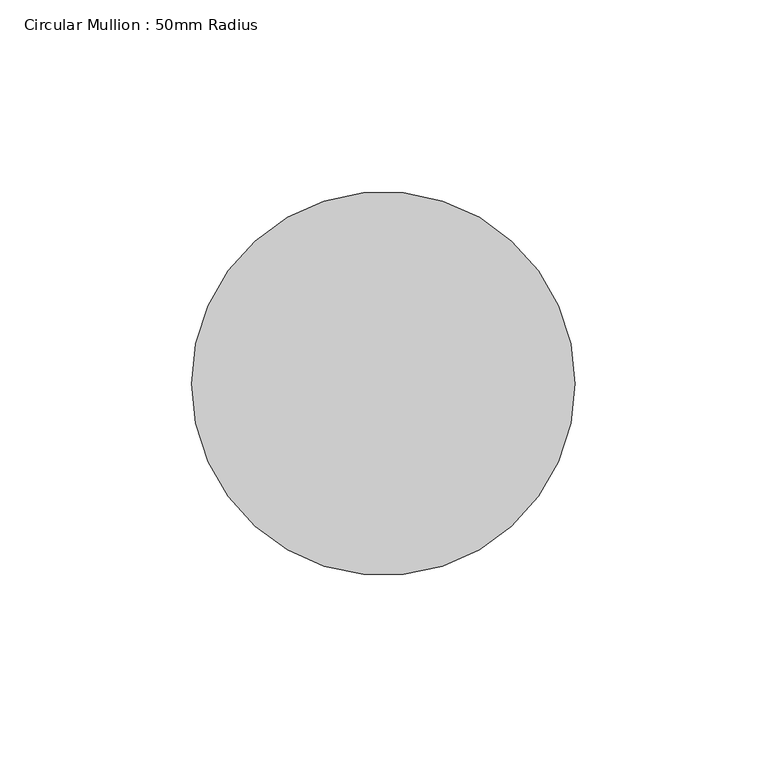
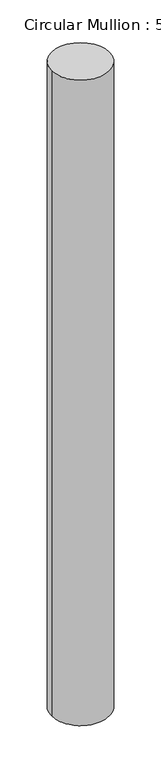
"""IFC4 building model written with IfcOpenShell, lengths in millimetres: member geometry, Circular Mullion : 50mm Radius."""

from ifc_helpers import new_model, si_unit, frame, origin, place, context, project, spatial, ellipse_curve, source, transform, mapped, element, save
from ifc_brep_helpers import plane_surface, cylinder_surface, advanced_brep


def circular_mullion_50mm_radius_35edecd0(model_context):
    return source(origin(), model_context, "Body", "AdvancedBrep", [
        advanced_brep(
        [(-100.0, 0.0, 0.7649818), (0.0, 0.0, 0.0), (0.0, 0.0, -1179.5961113), (-100.0, 0.0, -1180.3293723)],
        [
            (0, 1, ellipse_curve(frame((-50.0, 0.0, 0.3824909), z_axis=(-0.007648899186125256, -0.013483113711122539, -0.9998798427740673), x_axis=(-0.49336672127457615, -0.8696832632198164, 0.015501613274313146)), 50.0060086, 50.0)),
            (1, 2),
            (2, 3, ellipse_curve(frame((-50.0, 0.0, -1179.9627418), z_axis=(-0.0073318009043386, -0.012924148023788112, 0.9998895994525389), x_axis=(0.49337153547347923, 0.8696917494594852, 0.014858967213143224)), 50.0055206, 50.0)),
            (3, 0),
            (1, 0, ellipse_curve(frame((-50.0, 0.0, 0.3824909), z_axis=(-0.007648899186125256, -0.013483113711122539, -0.9998798427740673), x_axis=(-0.49336672127457615, -0.8696832632198164, 0.015501613274313146)), 50.0060086, 50.0)),
            (3, 2, ellipse_curve(frame((-50.0, 0.0, -1179.9627418), z_axis=(-0.0073318009043386, -0.012924148023788112, 0.9998895994525389), x_axis=(0.49337153547347923, 0.8696917494594852, 0.014858967213143224)), 50.0055206, 50.0)),
        ],
        [
            cylinder_surface(frame((-50.0, 0.0, 0.0), z_axis=(0.0, 0.0, 1.0), x_axis=(1.0, 0.0, 0.0)), 50.0),
            plane_surface(frame((-265.1113137, 150.3962478, 0.0), z_axis=(0.007648899186125256, 0.013483113711122539, 0.9998798427740673), x_axis=(0.4933667212745753, 0.8696832632198167, -0.015501613274319813))),
            plane_surface(frame((-265.1113137, 150.3962478, -1179.5961113), z_axis=(0.0073318009043386, 0.012924148023788112, -0.9998895994525389), x_axis=(0.4933715354734791, 0.8696917494594852, 0.014858967213156049))),
        ],
        [
            (0, [[1, 2, 3, 4]]),
            (0, [[5, -4, 6, -2]]),
            (1, [[-1, -5]]),
            (2, [[-6, -3]]),
        ],
    ),
    ])


if __name__ == "__main__":
    model = new_model("IFC4")
    model_context = context("Model", 3, world=origin())
    ifc_project = project(units=[si_unit("LENGTHUNIT", "METRE", prefix="MILLI")], contexts=[model_context])
    site = spatial("IfcSite", under=ifc_project)
    building = spatial("IfcBuilding", under=site)
    placement = place(None, origin())
    circular_mullion_50mm_radius_shape = circular_mullion_50mm_radius_35edecd0(model_context)
    element("IfcMember", 1, ObjectType="Circular Mullion : 50mm Radius", at=placement, inside=building, context=model_context, shape_type="MappedRepresentation", body=[
        mapped(circular_mullion_50mm_radius_shape, transform((0.0, 0.0, 0.0), x_axis=(1.0, 0.0, 0.0), y_axis=(0.0, 1.0, 0.0), z_axis=(0.0, 0.0, 1.0))),
    ])
    save(model, "model.ifc")

# Revit data of these elements
# Type "Circular Mullion : 50mm Radius"
#   built-in parameter 1007350 = 0.164042 (stored number, unit not read)
# Element 1 (IfcMember, "Circular Mullion : 50mm Radius")
#   Materials on its faces: "Aluminium"
# Materials
#   "Aluminium": class "Metal", colour RGB 247 247 247, transparency 0, Description = "Aluminium 6061", Cost = 0
